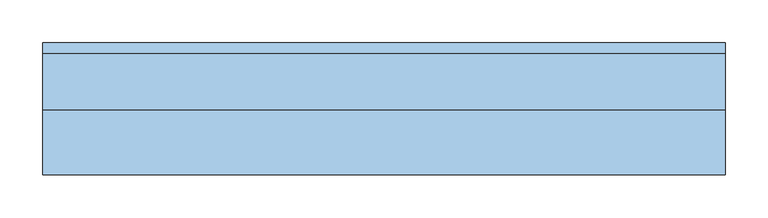
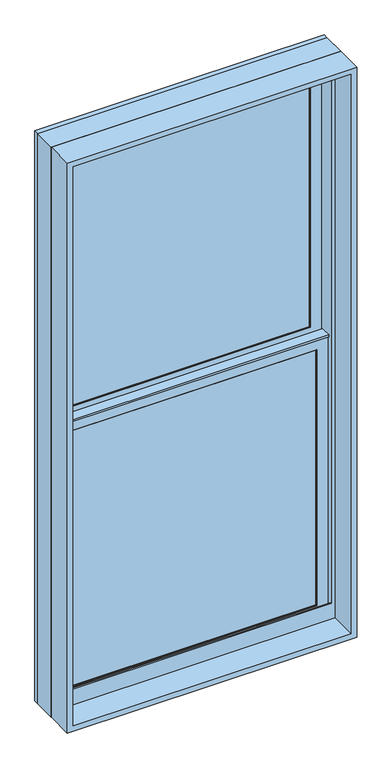
"""IFC4 building model written with IfcOpenShell, lengths in millimetres: window geometry, Window-Double_Hung-Marvin-Essential : ESDH2856."""

from ifc_helpers import new_model, si_unit, frame, origin, place, context, project, spatial, polyline, outline, extrude, faceted_brep, source, transform, mapped, element, save


def window_3446b1fa(model_context):
    return source(origin(), model_context, "Body", "SolidModel", [
        extrude(outline(polyline([(123.825, 20.6375), (123.825, 15.875), (104.775, 15.875), (104.775, 20.6375), (123.825, 20.6375)])), frame((0.0, 0.0, 831.85), z_axis=(0.0, 0.0, 1.0), x_axis=(1.0, 0.0, 0.0)), (0.0, 0.0, 1.0), 755.65),
        extrude(outline(polyline([(-104.775, 20.6375), (-104.775, 15.875), (-123.825, 15.875), (-123.825, 20.6375), (-104.775, 20.6375)])), frame((0.0, 0.0, 831.85), z_axis=(0.0, 0.0, 1.0), x_axis=(1.0, 0.0, 0.0)), (0.0, 0.0, 1.0), 755.65),
        extrude(outline(polyline([(342.9, 20.6375), (342.9, 15.875), (-342.9, 15.875), (-342.9, 20.6375), (342.9, 20.6375)])), frame((0.0, 0.0, 1200.15), z_axis=(0.0, 0.0, 1.0), x_axis=(1.0, 0.0, 0.0)), (0.0, 0.0, 1.0), 19.05),
        extrude(outline(polyline([(-123.825, 46.83125), (-123.825, 51.59375), (-104.775, 51.59375), (-104.775, 46.83125), (-123.825, 46.83125)])), frame((0.0, 0.0, 1625.6), z_axis=(0.0, 0.0, 1.0), x_axis=(1.0, 0.0, 0.0)), (0.0, 0.0, 1.0), 755.65),
        extrude(outline(polyline([(104.775, 46.83125), (104.775, 51.59375), (123.825, 51.59375), (123.825, 46.83125), (104.775, 46.83125)])), frame((0.0, 0.0, 1625.6), z_axis=(0.0, 0.0, 1.0), x_axis=(1.0, 0.0, 0.0)), (0.0, 0.0, 1.0), 755.65),
        extrude(outline(polyline([(-342.9, 46.83125), (-342.9, 51.59375), (342.9, 51.59375), (342.9, 46.83125), (-342.9, 46.83125)])), frame((0.0, 0.0, 1993.9), z_axis=(0.0, 0.0, 1.0), x_axis=(1.0, 0.0, 0.0)), (0.0, 0.0, 1.0), 19.05),
        extrude(outline(polyline([(123.825, 20.6375), (104.775, 20.6375), (104.775, 25.4), (123.825, 25.4), (123.825, 20.6375)])), frame((0.0, 0.0, 831.85), z_axis=(0.0, 0.0, 1.0), x_axis=(1.0, 0.0, 0.0)), (0.0, 0.0, 1.0), 755.65),
        extrude(outline(polyline([(-104.775, 20.6375), (-123.825, 20.6375), (-123.825, 25.4), (-104.775, 25.4), (-104.775, 20.6375)])), frame((0.0, 0.0, 831.85), z_axis=(0.0, 0.0, 1.0), x_axis=(1.0, 0.0, 0.0)), (0.0, 0.0, 1.0), 755.65),
        extrude(outline(polyline([(342.9, 20.6375), (-342.9, 20.6375), (-342.9, 25.4), (342.9, 25.4), (342.9, 20.6375)])), frame((0.0, 0.0, 1200.15), z_axis=(0.0, 0.0, 1.0), x_axis=(1.0, 0.0, 0.0)), (0.0, 0.0, 1.0), 19.05),
        extrude(outline(polyline([(-123.825, 56.35625), (-104.775, 56.35625), (-104.775, 51.59375), (-123.825, 51.59375), (-123.825, 56.35625)])), frame((0.0, 0.0, 1625.6), z_axis=(0.0, 0.0, 1.0), x_axis=(1.0, 0.0, 0.0)), (0.0, 0.0, 1.0), 755.65),
        extrude(outline(polyline([(104.775, 56.35625), (123.825, 56.35625), (123.825, 51.59375), (104.775, 51.59375), (104.775, 56.35625)])), frame((0.0, 0.0, 1625.6), z_axis=(0.0, 0.0, 1.0), x_axis=(1.0, 0.0, 0.0)), (0.0, 0.0, 1.0), 755.65),
        extrude(outline(polyline([(-342.9, 56.35625), (342.9, 56.35625), (342.9, 51.59375), (-342.9, 51.59375), (-342.9, 56.35625)])), frame((0.0, 0.0, 1993.9), z_axis=(0.0, 0.0, 1.0), x_axis=(1.0, 0.0, 0.0)), (0.0, 0.0, 1.0), 19.05),
        faceted_brep([(-369.8875, 5.6780605, 1617.5351748), (-369.8875, 5.6780605, 1612.9), (369.8875, 5.6780605, 1612.9), (369.8875, 5.6780605, 1617.5351748), (-369.8875, 34.8118605, 1617.5351748), (369.8875, 34.8118605, 1617.5351748), (369.8875, 34.8118605, 1612.9), (-369.8875, 34.8118605, 1612.9), (-369.8875, 30.1625, 1612.9), (-369.8875, 30.1625, 804.8625), (-369.8875, 8.9241104, 804.8625), (-369.8875, 8.9241104, 1612.9), (369.8875, 8.9241104, 1612.9), (369.8875, 30.1625, 1612.9), (369.8875, 8.9241104, 804.8625), (369.8875, 30.1625, 804.8625), (-354.0034752, 11.90625, 1598.6034752), (-354.0034752, 30.1625, 1598.6034752), (354.0034752, 30.1625, 1598.6034752), (354.0034752, 11.90625, 1598.6034752), (-337.34375, 10.4662439, 1581.94375), (-337.34375, 11.90625, 1581.94375), (337.34375, 11.90625, 1581.94375), (337.34375, 10.4662439, 1581.94375), (338.8858834, 8.9241104, 1583.4858834), (-338.8858834, 8.9241104, 1583.4858834), (354.0034752, 30.1625, 820.7465248), (354.0034752, 11.90625, 820.7465248), (337.34375, 11.90625, 837.40625), (337.34375, 10.4662439, 837.40625), (338.8858834, 8.9241104, 835.8641166), (-354.0034752, 30.1625, 820.7465248), (-354.0034752, 11.90625, 820.7465248), (-337.34375, 11.90625, 837.40625), (-337.34375, 10.4662439, 837.40625), (-338.8858834, 8.9241104, 835.8641166)], [[[0, 1, 2, 3]], [[4, 5, 6, 7]], [[1, 0, 4, 7, 8, 9, 10, 11]], [[2, 1, 11, 12]], [[7, 6, 13, 8]], [[3, 2, 12, 14, 15, 13, 6, 5]], [[0, 3, 5, 4]], [[16, 17, 18, 19]], [[20, 21, 22, 23]], [[20, 23, 24, 25]], [[19, 18, 26, 27]], [[23, 22, 28, 29]], [[24, 23, 29, 30]], [[27, 26, 31, 32]], [[29, 28, 33, 34]], [[30, 29, 34, 35]], [[15, 14, 10, 9]], [[15, 9, 8, 13], [18, 17, 31, 26]], [[17, 16, 32, 31]], [[16, 19, 27, 32], [22, 21, 33, 28]], [[21, 20, 34, 33]], [[20, 25, 35, 34]], [[10, 14, 12, 11], [25, 24, 30, 35]]]),
        extrude(outline(polyline([(38.5955581, 1598.6125), (33.5778968, 1598.6125), (33.5778968, 1600.2), (39.9405976, 1600.2), (39.9405976, 1598.6125), (61.515625, 1598.6125), (47.6307501, 1595.2975159), (38.5955581, 1595.2975159), (38.5955581, 1598.6125)])), frame((-369.8875, 0.0, 0.0), z_axis=(1.0, 0.0, 0.0), x_axis=(0.0, 1.0, 0.0)), (0.0, 0.0, 1.0), 739.775),
        faceted_brep([(400.05, 0.0, 774.7), (400.05, 0.0, 2438.4), (-400.05, 0.0, 2438.4), (-400.05, 0.0, 774.7), (373.85625, 0.0, 835.81875), (-373.85625, 0.0, 835.81875), (-373.85625, 0.0, 2412.20625), (373.85625, 0.0, 2412.20625), (373.85625, 3.96875, 774.7), (-373.85625, 3.96875, 774.7), (-373.85625, 3.96875, 835.81875), (373.85625, 3.96875, 835.81875), (-400.05, 65.6828125, 774.7), (-373.85625, 65.6828125, 774.7), (373.85625, 65.6828125, 774.7), (400.05, 65.6828125, 774.7), (-400.05, 65.6828125, 2438.4), (400.05, 65.6828125, 2438.4), (373.85625, 65.6828125, 2412.20625), (-373.85625, 65.6828125, 2412.20625)], [[[0, 1, 2, 3], [4, 5, 6, 7]], [[8, 9, 10, 11]], [[5, 4, 11, 10]], [[0, 3, 12, 13, 9, 8, 14, 15]], [[13, 12, 16, 17, 15, 14, 18, 19]], [[13, 19, 6, 5, 10, 9]], [[7, 6, 19, 18]], [[18, 14, 8, 11, 4, 7]], [[1, 0, 15, 17]], [[2, 1, 17, 16]], [[3, 2, 16, 12]]]),
        faceted_brep([(373.85625, 30.1625, 1606.55), (372.26875, 30.1625, 1606.55), (372.26875, 30.1625, 799.0544613), (373.85625, 30.1625, 799.0544613), (-372.26875, 30.1625, 1606.55), (-373.85625, 30.1625, 1606.55), (-373.85625, 30.1625, 799.0544613), (-372.26875, 30.1625, 799.0544613), (372.26875, 63.5, 1606.55), (373.85625, 63.5, 1606.55), (373.85625, 63.5, 792.5743077), (372.26875, 63.5, 792.5743077), (-373.85625, 63.5, 1606.55), (-372.26875, 63.5, 1606.55), (-372.26875, 63.5, 792.5743077), (-373.85625, 63.5, 792.5743077), (385.1108932, 3.96875, 804.1460105), (385.1108932, 3.96875, 774.7), (385.1108932, 65.6828125, 774.7), (385.1108932, 65.6828125, 792.150012), (-385.1108932, 3.96875, 774.7), (-385.1108932, 3.96875, 804.1460105), (-385.1108932, 65.6828125, 792.150012), (-385.1108932, 65.6828125, 774.7), (385.1108932, 78.58125, 789.6428097), (-385.1108932, 78.58125, 789.6428097), (-383.0971252, 68.2348864, 791.6539391), (-365.13135, 68.2348864, 791.6539391), (-365.13135, 65.6828125, 792.150012), (365.13135, 65.6828125, 792.150012), (365.13135, 68.2348864, 791.6539391), (383.0971252, 68.2348864, 791.6539391), (-400.05, 65.6828125, 774.7), (-400.05, 78.5948249, 774.7), (400.05, 78.5948249, 774.7), (400.05, 65.6828125, 774.7), (-400.05, 78.58125, 2438.4), (400.05, 78.58125, 2438.4), (385.1108932, 78.58125, 2423.4608932), (-385.1108932, 78.58125, 2423.4608932), (-400.05, 65.6828125, 2438.4), (-383.0971252, 68.2348864, 2421.4471252), (383.0971252, 68.2348864, 2421.4471252), (365.13135, 68.2348864, 2403.48135), (-365.13135, 68.2348864, 2403.48135), (-365.13135, 65.6828125, 2403.48135), (365.13135, 65.6828125, 2403.48135), (400.05, 65.6828125, 2438.4)], [[[0, 1, 2, 3]], [[4, 5, 6, 7]], [[8, 9, 10, 11]], [[12, 13, 14, 15]], [[1, 8, 11, 2]], [[9, 0, 3, 10]], [[1, 0, 9, 8]], [[5, 4, 13, 12]], [[5, 12, 15, 6]], [[13, 4, 7, 14]], [[16, 17, 18, 19]], [[20, 21, 22, 23]], [[24, 25, 26, 27, 28, 22, 21, 16, 19, 29, 30, 31], [3, 2, 11, 10], [7, 6, 15, 14]], [[17, 16, 21, 20]], [[17, 20, 23, 32, 33, 34, 35, 18]], [[34, 33, 36, 37], [25, 24, 38, 39]], [[33, 32, 40, 36]], [[39, 41, 26, 25]], [[41, 42, 31, 30, 43, 44, 27, 26]], [[44, 45, 28, 27]], [[40, 32, 23, 22, 28, 45, 46, 29, 19, 18, 35, 47]], [[36, 40, 47, 37]], [[39, 38, 42, 41]], [[44, 43, 46, 45]], [[34, 37, 47, 35]], [[42, 38, 24, 31]], [[46, 43, 30, 29]]]),
        extrude(outline(polyline([(350.04375, 11.90625), (-350.04375, 11.90625), (-350.04375, 15.08125), (350.04375, 15.08125), (350.04375, 11.90625)])), frame((0.0, 0.0, 824.70625), z_axis=(0.0, 0.0, 1.0), x_axis=(1.0, 0.0, 0.0)), (0.0, 0.0, 1.0), 769.9375),
        extrude(outline(polyline([(350.04375, 42.8625), (-350.04375, 42.8625), (-350.04375, 46.0375), (350.04375, 46.0375), (350.04375, 42.8625)])), frame((0.0, 0.0, 1618.45625), z_axis=(0.0, 0.0, 1.0), x_axis=(1.0, 0.0, 0.0)), (0.0, 0.0, 1.0), 769.9375),
        faceted_brep([(-337.34375, 31.194477, 1581.94375), (-338.8858834, 32.7366104, 1583.4858834), (338.8858834, 32.7366104, 1583.4858834), (337.34375, 31.194477, 1581.94375), (-337.34375, 30.1625, 1581.94375), (337.34375, 30.1625, 1581.94375), (-369.8875, 32.7366104, 1614.4875), (-369.8875, 30.1625, 1614.4875), (369.8875, 30.1625, 1614.4875), (369.8875, 32.7366104, 1614.4875), (338.8858834, 32.7366104, 835.8641166), (337.34375, 31.194477, 837.40625), (337.34375, 30.1625, 837.40625), (369.8875, 30.1625, 804.8625), (369.8875, 32.7366104, 804.8625), (-338.8858834, 32.7366104, 835.8641166), (-337.34375, 31.194477, 837.40625), (-337.34375, 30.1625, 837.40625), (-369.8875, 30.1625, 804.8625), (-369.8875, 32.7366104, 804.8625)], [[[0, 1, 2, 3]], [[4, 0, 3, 5]], [[6, 7, 8, 9]], [[3, 2, 10, 11]], [[5, 3, 11, 12]], [[9, 8, 13, 14]], [[11, 10, 15, 16]], [[12, 11, 16, 17]], [[14, 13, 18, 19]], [[9, 14, 19, 6], [1, 15, 10, 2]], [[16, 15, 1, 0]], [[17, 16, 0, 4]], [[7, 18, 13, 8], [5, 12, 17, 4]], [[19, 18, 7, 6]]]),
        faceted_brep([(-354.0034752, 42.8625, 2392.3534752), (-354.0034752, 61.11875, 2392.3534752), (354.0034752, 61.11875, 2392.3534752), (354.0034752, 42.8625, 2392.3534752), (-337.34375, 41.4224939, 2375.69375), (-337.34375, 42.8625, 2375.69375), (337.34375, 42.8625, 2375.69375), (337.34375, 41.4224939, 2375.69375), (-338.8858834, 39.8803604, 2377.2358834), (338.8858834, 39.8803604, 2377.2358834), (-369.8875, 61.11875, 2408.2375), (-369.8875, 39.8803604, 2408.2375), (369.8875, 39.8803604, 2408.2375), (369.8875, 61.11875, 2408.2375), (354.0034752, 61.11875, 1614.4965248), (354.0034752, 42.8625, 1614.4965248), (337.34375, 42.8625, 1631.15625), (337.34375, 41.4224939, 1631.15625), (338.8858834, 39.8803604, 1629.6141166), (369.8875, 39.8803604, 1598.6125), (369.8875, 61.11875, 1598.6125), (-354.0034752, 61.11875, 1614.4965248), (-354.0034752, 42.8625, 1614.4965248), (-337.34375, 42.8625, 1631.15625), (-337.34375, 41.4224939, 1631.15625), (-338.8858834, 39.8803604, 1629.6141166), (-369.8875, 39.8803604, 1598.6125), (-369.8875, 61.11875, 1598.6125)], [[[0, 1, 2, 3]], [[4, 5, 6, 7]], [[8, 4, 7, 9]], [[10, 11, 12, 13]], [[3, 2, 14, 15]], [[7, 6, 16, 17]], [[9, 7, 17, 18]], [[13, 12, 19, 20]], [[15, 14, 21, 22]], [[17, 16, 23, 24]], [[18, 17, 24, 25]], [[20, 19, 26, 27]], [[13, 20, 27, 10], [1, 21, 14, 2]], [[22, 21, 1, 0]], [[3, 15, 22, 0], [5, 23, 16, 6]], [[24, 23, 5, 4]], [[25, 24, 4, 8]], [[11, 26, 19, 12], [9, 18, 25, 8]], [[27, 26, 11, 10]]]),
        faceted_brep([(-369.8875, 61.11875, 1598.6125), (-369.8875, 63.6928604, 1598.6125), (369.8875, 63.6928604, 1598.6125), (369.8875, 61.11875, 1598.6125), (-337.34375, 62.150727, 1631.15625), (-337.34375, 61.11875, 1631.15625), (337.34375, 61.11875, 1631.15625), (337.34375, 62.150727, 1631.15625), (-338.8858834, 63.6928604, 1629.6141166), (338.8858834, 63.6928604, 1629.6141166), (369.8875, 63.6928604, 2408.2375), (369.8875, 61.11875, 2408.2375), (337.34375, 61.11875, 2375.69375), (337.34375, 62.150727, 2375.69375), (338.8858834, 63.6928604, 2377.2358834), (-369.8875, 63.6928604, 2408.2375), (-369.8875, 61.11875, 2408.2375), (-337.34375, 61.11875, 2375.69375), (-337.34375, 62.150727, 2375.69375), (-338.8858834, 63.6928604, 2377.2358834)], [[[0, 1, 2, 3]], [[4, 5, 6, 7]], [[8, 4, 7, 9]], [[3, 2, 10, 11]], [[7, 6, 12, 13]], [[9, 7, 13, 14]], [[11, 10, 15, 16]], [[13, 12, 17, 18]], [[14, 13, 18, 19]], [[16, 15, 1, 0]], [[3, 11, 16, 0], [5, 17, 12, 6]], [[18, 17, 5, 4]], [[19, 18, 4, 8]], [[1, 15, 10, 2], [9, 14, 19, 8]]]),
        extrude(outline(polyline([(350.04375, 26.19375), (-350.04375, 26.19375), (-350.04375, 30.1625), (350.04375, 30.1625), (350.04375, 26.19375)])), frame((0.0, 0.0, 824.70625), z_axis=(0.0, 0.0, 1.0), x_axis=(1.0, 0.0, 0.0)), (0.0, 0.0, 1.0), 769.9375),
        extrude(outline(polyline([(350.04375, 57.15), (-350.04375, 57.15), (-350.04375, 61.11875), (350.04375, 61.11875), (350.04375, 57.15)])), frame((0.0, 0.0, 1618.45625), z_axis=(0.0, 0.0, 1.0), x_axis=(1.0, 0.0, 0.0)), (0.0, 0.0, 1.0), 769.9375),
        extrude(outline(polyline([(2438.4, 400.05), (2438.4, -400.05), (774.7, -400.05), (774.7, 400.05), (2438.4, 400.05)]), holes=[polyline([(2422.525, 384.175), (790.575, 384.175), (790.575, -384.175), (2422.525, -384.175), (2422.525, 384.175)])]), frame((0.0, -76.2, 0.0), z_axis=(0.0, 1.0, 0.0), x_axis=(0.0, 0.0, 1.0)), (0.0, 0.0, 1.0), 75.40625),
    ])


if __name__ == "__main__":
    model = new_model("IFC4")
    model_context = context("Model", 3, world=origin())
    ifc_project = project(units=[si_unit("LENGTHUNIT", "METRE", prefix="MILLI")], contexts=[model_context])
    site = spatial("IfcSite", under=ifc_project)
    building = spatial("IfcBuilding", under=site)
    placement = place(None, origin())
    window_shape = window_3446b1fa(model_context)
    element("IfcWindow", 1, ObjectType="Window-Double_Hung-Marvin-Essential : ESDH2856", at=placement, inside=building, context=model_context, shape_type="MappedRepresentation", body=[
        mapped(window_shape, transform((0.0, 0.0, 0.0), x_axis=(1.0, 0.0, 0.0), y_axis=(0.0, 1.0, 0.0), z_axis=(0.0, 0.0, 1.0))),
    ])
    save(model, "model.ifc")

# Revit data of these elements
# Type "Window-Double_Hung-Marvin-Essential : ESDH2856"
#   Type Mark = "71"
#   Window Type = "Essential Double Hung"
#   Product data url = "https://bimobject.com/marvin-windows-and-doors/product/marvin-dhwau"
#   Product Guid = "c4a96547-874c-4385-91dc-a058adc19d98"
#   Frame = "All Ultrex"
#   Egress Window = "No"
#   URL = "www.marvin.com"
#   Model = "ESDH2856"
#   Manufacturer = "Marvin Windows and Doors"
#   Label Egress = ""
#   Glass Type = "IG Low E II with Argon"
#   Design Pressure = "DP40"
#   Description = "3266 DBHG"
#   Analytic Construction = "<None>"
#   Prairie Corner Width = 0' - 4"
#   Prairie Corner Height = 0' - 4"
#   Egress Width = 2' - 4 9/16"
#   Egress Height = 2' - 4 27/128"
#   Rough Width = 2' - 8"
#   Rough Height = 5' - 6"
#   Nominal Width = 2' - 8"
#   Nominal Height = 5' - 6"
#   Inset to Installation Flange [instance default] = 0' - 1"
#   Height = 5' - 5 1/2"
#   Egress Area = 5.59566 SF
#   Default Head Height = 8' - 0"
#   Width = 2' - 7 1/2"
#   Daylight Area = 10.8141 SF
#   DLO Width = 2' - 2 9/16"
#   DLO Height = 2' - 5 5/16"
#   Muntins Top Sash = yes
#   Lites Wide Top Sash = 3
#   Lites Wide Bottom Sash = 3
#   Lites High Top Sash = 2
#   Lites High Bottom Sash = 2
#   Lite Cut Prairie 9 = no
#   Lite Cut HV Grid = yes
#   Muntins Bottom Sash = yes
#   Label Visibility = no
#   Jamb Extension Visibility = yes
#   Edition number = 1
#   Interior Material = Ultrex-Marvin-Stonewhite
#   Glazing Material = Glass-Marvin-IG Low E II with Argon
#   Cladding Material = Ultrex-Marvin-Pebblegray
#   Wall Closure = (empty or 0)
#   Assembly Code = ""
# Element 1 (IfcWindow, "Window-Double_Hung-Marvin-Essential : ESDH2856")
#   Materials on its faces: "Ultrex-Marvin-Pebblegray", "Ultrex-Marvin-Stonewhite", "Glass-Marvin-IG Low E II with Argon"
# Materials
#   "Ultrex-Marvin-Stonewhite": class "Paint", colour RGB 250 251 245, transparency 0
#   "Glass-Marvin-IG Low E II with Argon": class "Glass", colour RGB 0 128 192, transparency 0.85
#   "Ultrex-Marvin-Pebblegray": class "Paint", colour RGB 189 185 173, transparency 0
